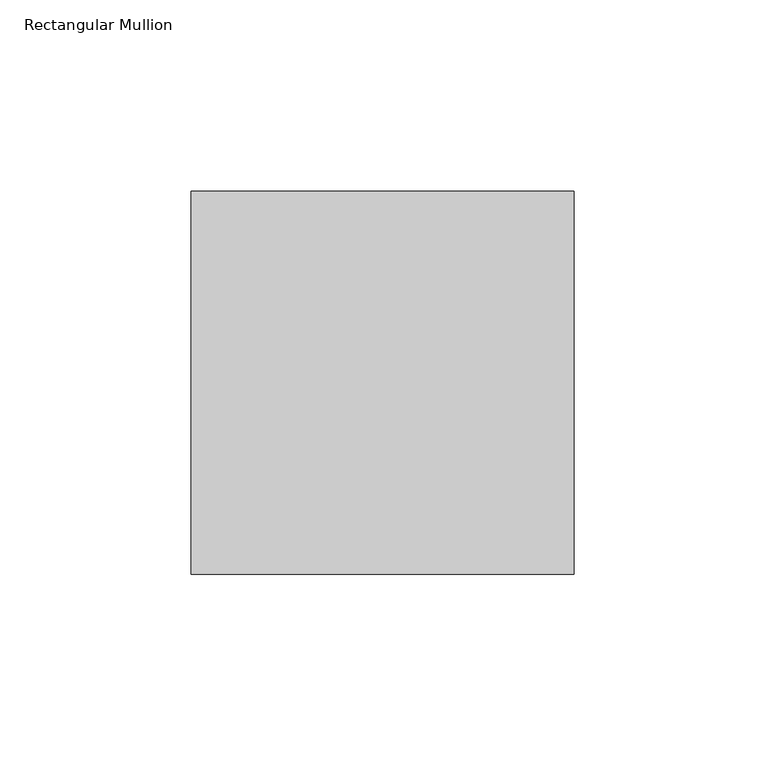
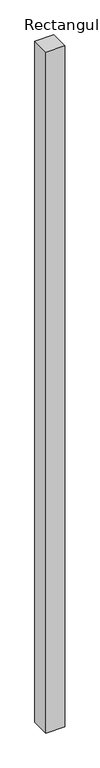
"""IFC4 building model written with IfcOpenShell, lengths in millimetres: member geometry, Rectangular Mullion : 알루미늄_Rectangular Cap_100 x100."""

import ifcopenshell
import ifcopenshell.guid

model = None  # the IFC model being written
_history = None  # IfcOwnerHistory: only IFC2X3 demands one
_inside = {}  # id of a spatial element -> (the spatial element, [elements in it])
_under = {}  # id of a project, library or spatial element -> (it, [spatial elements below it])
_declared = {}  # id of a project -> (the project, [libraries it declares])
_typed = {}  # id of a type object -> (the type object, [elements of that type])
_made_of = {}  # id of a material, layer set ... -> (it, [elements and type objects made of it])


def new_model(schema):
    """Start an empty IFC model of exactly this schema.

    Asked for "IFC4X3", IfcOpenShell would pick the latest addendum, in which some entities
    have other attributes; the version numbers below select the first issue.
    IFC2X3 requires an IfcOwnerHistory on every rooted entity: one is made here for all.
    """
    global model, _history
    if schema == "IFC4X3":
        model = ifcopenshell.file(schema_version=(4, 3, 0, 0))
    else:
        model = ifcopenshell.file(schema=schema)
    _inside.clear()
    _under.clear()
    _declared.clear()
    _typed.clear()
    _made_of.clear()
    _history = None
    if model.schema == "IFC2X3":
        org = make("IfcOrganization", Name="unknown")
        user = make(
            "IfcPersonAndOrganization",
            ThePerson=make("IfcPerson", FamilyName="unknown"),
            TheOrganization=org,
        )
        app = make(
            "IfcApplication",
            ApplicationDeveloper=org,
            Version="unknown",
            ApplicationFullName="unknown",
            ApplicationIdentifier="unknown",
        )
        _history = make(
            "IfcOwnerHistory",
            OwningUser=user,
            OwningApplication=app,
            ChangeAction="ADDED",
            CreationDate=0,
        )
    return model


def make(cls, **values):
    """One entity of the class cls with the attributes given. An attribute that is None is left unset."""
    return model.create_entity(
        cls, **{name: value for name, value in values.items() if value is not None}
    )


def rooted(cls, **values):
    """An entity with a GlobalId (a new one), such as an element, a storey or a relation."""
    return make(cls, GlobalId=ifcopenshell.guid.new(), OwnerHistory=_history, **values)


def si_unit(unit_type, name, prefix=None):
    """IfcSIUnit, for example si_unit("LENGTHUNIT", "METRE", prefix="MILLI")."""
    return make("IfcSIUnit", UnitType=unit_type, Prefix=prefix, Name=name)


def assignment(units):
    """IfcUnitAssignment: the units of a project."""
    return None if units is None else make("IfcUnitAssignment", Units=units)


def point(xyz):
    """IfcCartesianPoint."""
    return None if xyz is None else make("IfcCartesianPoint", Coordinates=xyz)


def direction(xyz):
    """IfcDirection."""
    return None if xyz is None else make("IfcDirection", DirectionRatios=xyz)


def frame(location, z_axis=None, x_axis=None):
    """IfcAxis2Placement3D, a coordinate frame: its origin and axes. An axis left out is left unset."""
    return make(
        "IfcAxis2Placement3D",
        Location=point(location),
        Axis=direction(z_axis),
        RefDirection=direction(x_axis),
    )


def origin():
    """The frame at (0, 0, 0) with its axes left unset."""
    return frame((0.0, 0.0, 0.0))


def place(relative_to, where):
    """IfcLocalPlacement: puts the frame where relative to a parent placement (None: the world)."""
    return make(
        "IfcLocalPlacement", PlacementRelTo=relative_to, RelativePlacement=where
    )


def context(
    kind, dimensions, precision=None, world=None, true_north=None, identifier=None
):
    """IfcGeometricRepresentationContext, for example the 3D "Model" context."""
    return make(
        "IfcGeometricRepresentationContext",
        ContextIdentifier=identifier,
        ContextType=kind,
        CoordinateSpaceDimension=dimensions,
        Precision=precision,
        WorldCoordinateSystem=world,
        TrueNorth=true_north,
    )


def project(units=None, contexts=None):
    """IfcProject with its units and contexts."""
    return rooted(
        "IfcProject",
        Name="project",
        RepresentationContexts=contexts,
        UnitsInContext=assignment(units),
    )


def spatial(cls, under=None, at=None, **own):
    """A site, building, storey or space (cls), placed at a placement, below another one or the project."""
    s = rooted(cls, ObjectPlacement=at, **own)
    if under is not None:
        _under.setdefault(under.id(), (under, []))[1].append(s)
    return s


def polyline(points):
    """IfcPolyline through the points."""
    return make("IfcPolyline", Points=[point(p) for p in points])


def outline(outer, holes=None, kind="AREA"):
    """IfcArbitraryClosedProfileDef: a profile drawn as a closed curve; with holes, ...WithVoids."""
    if holes is None:
        return make("IfcArbitraryClosedProfileDef", ProfileType=kind, OuterCurve=outer)
    return make(
        "IfcArbitraryProfileDefWithVoids",
        ProfileType=kind,
        OuterCurve=outer,
        InnerCurves=holes,
    )


def extrude(swept, where, along, depth):
    """IfcExtrudedAreaSolid: the profile swept, set in the frame where, extruded along a direction by depth."""
    return make(
        "IfcExtrudedAreaSolid",
        SweptArea=swept,
        Position=where,
        ExtrudedDirection=direction(along),
        Depth=depth,
    )


def shape(context_of_items, identifier, shape_type, items):
    """IfcShapeRepresentation: the items that make up one representation, for example the "Body"."""
    return make(
        "IfcShapeRepresentation",
        ContextOfItems=context_of_items,
        RepresentationIdentifier=identifier,
        RepresentationType=shape_type,
        Items=items,
    )


def source(mapping_origin, context_of_items, identifier, shape_type, items):
    """IfcRepresentationMap: a shape defined once, which mapped items show again and again."""
    return make(
        "IfcRepresentationMap",
        MappingOrigin=mapping_origin,
        MappedRepresentation=shape(context_of_items, identifier, shape_type, items),
    )


def transform(
    local_origin,
    x_axis=None,
    y_axis=None,
    z_axis=None,
    scale=None,
    scale2=None,
    scale3=None,
    uniform=True,
):
    """IfcCartesianTransformationOperator3D, or its non-uniform kind. x_axis, y_axis, z_axis: its Axis1, 2, 3."""
    if uniform:
        return make(
            "IfcCartesianTransformationOperator3D",
            Axis1=direction(x_axis),
            Axis2=direction(y_axis),
            LocalOrigin=point(local_origin),
            Scale=scale,
            Axis3=direction(z_axis),
        )
    return make(
        "IfcCartesianTransformationOperator3DnonUniform",
        Axis1=direction(x_axis),
        Axis2=direction(y_axis),
        LocalOrigin=point(local_origin),
        Scale=scale,
        Axis3=direction(z_axis),
        Scale2=scale2,
        Scale3=scale3,
    )


def mapped(mapping_source, mapping_target):
    """IfcMappedItem: shows the shape of a source again, moved by a transform."""
    return make(
        "IfcMappedItem", MappingSource=mapping_source, MappingTarget=mapping_target
    )


def made_of(thing, what):
    """Note that an element or type object is made of a material, layer set ...; save() writes the relation."""
    if what is not None:
        _made_of.setdefault(what.id(), (what, []))[1].append(thing)
    return thing


def element(
    cls,
    number,
    at=None,
    inside=None,
    cuts=None,
    type_object=None,
    material=None,
    context=None,
    identifier="Body",
    shape_type=None,
    held_by="IfcProductDefinitionShape",
    body=None,
    shapes=None,
    **own,
):
    """One element of the class cls, such as IfcWall. Its Tag is "e" and its number.

    at: its placement. inside: the storey or other place that contains it. cuts: it is an
    opening in that element (IfcRelVoidsElement). A single representation is given by context,
    identifier, shape_type and body (its items); several are given by shapes. held_by: the class
    of the entity that holds the representations. save() writes the other relations.
    """
    e = rooted(cls, Tag="e%d" % number, ObjectPlacement=at, **own)
    if body is not None:
        shapes = [shape(context, identifier, shape_type, body)]
    if shapes is not None:
        e.Representation = make(held_by, Representations=shapes)
    if inside is not None:
        _inside.setdefault(inside.id(), (inside, []))[1].append(e)
    if cuts is not None:
        rooted(
            "IfcRelVoidsElement", RelatingBuildingElement=cuts, RelatedOpeningElement=e
        )
    if type_object is not None:
        _typed.setdefault(type_object.id(), (type_object, []))[1].append(e)
    return made_of(e, material)


def aggregate(whole, parts):
    """IfcRelAggregates: a whole, such as a stair, and the parts it consists of."""
    return rooted("IfcRelAggregates", RelatingObject=whole, RelatedObjects=parts)


def save(model, path):
    """Write the relations noted so far, then the file.

    IfcRelAggregates (storeys below a building ...), IfcRelContainedInSpatialStructure (elements
    in a storey), IfcRelDefinesByType, IfcRelAssociatesMaterial and IfcRelDeclares: one each for
    every whole, place, type object, material and project.
    """
    for whole, parts in _under.values():
        aggregate(whole, parts)
    for where, things in _inside.values():
        rooted(
            "IfcRelContainedInSpatialStructure",
            RelatedElements=things,
            RelatingStructure=where,
        )
    for kind, things in _typed.values():
        rooted("IfcRelDefinesByType", RelatedObjects=things, RelatingType=kind)
    for what, things in _made_of.values():
        rooted("IfcRelAssociatesMaterial", RelatedObjects=things, RelatingMaterial=what)
    for by, libraries in _declared.values():
        rooted("IfcRelDeclares", RelatingContext=by, RelatedDefinitions=libraries)
    model.write(path)


def rectangular_mullion_9ba7f3a8(model_context):
    return source(origin(), model_context, "Body", "SweptSolid", [
        extrude(outline(polyline([(0.0, 50.0), (0.0, -50.0), (-100.0, -50.0), (-100.0, 50.0), (0.0, 50.0)])), frame((0.0, 0.0, -3775.0), z_axis=(0.0, 0.0, 1.0), x_axis=(1.0, 0.0, 0.0)), (0.0, 0.0, 1.0), 3775.0),
    ])


if __name__ == "__main__":
    model = new_model("IFC4")
    model_context = context("Model", 3, world=origin())
    ifc_project = project(units=[si_unit("LENGTHUNIT", "METRE", prefix="MILLI")], contexts=[model_context])
    site = spatial("IfcSite", under=ifc_project)
    building = spatial("IfcBuilding", under=site)
    placement = place(None, origin())
    rectangular_mullion_shape = rectangular_mullion_9ba7f3a8(model_context)
    element("IfcMember", 1, ObjectType="Rectangular Mullion : 알루미늄_Rectangular Cap_100 x100", at=placement, inside=building, context=model_context, shape_type="MappedRepresentation", body=[
        mapped(rectangular_mullion_shape, transform((0.0, 0.0, 0.0), x_axis=(1.0, 0.0, 0.0), y_axis=(0.0, 1.0, 0.0), z_axis=(0.0, 0.0, 1.0))),
    ])
    save(model, "model.ifc")

# Revit data of these elements
# Type "Rectangular Mullion : 알루미늄_Rectangular Cap_100 x100"
#   built-in parameter 1007304 = 0.328084 (stored number, unit not read)
#   built-in parameter 1007301 = 0.164042 (stored number, unit not read)
#   built-in parameter 1007300 = 0.164042 (stored number, unit not read)
# Element 1 (IfcMember, "Rectangular Mullion : 알루미늄_Rectangular Cap_100 x100")
#   Materials on its faces: "00_Metal_Stainless Steel"
# Materials
#   "00_Metal_Stainless Steel": class "Metal", colour RGB 148 148 148, transparency 0, Description = "Steel", Cost = 0
